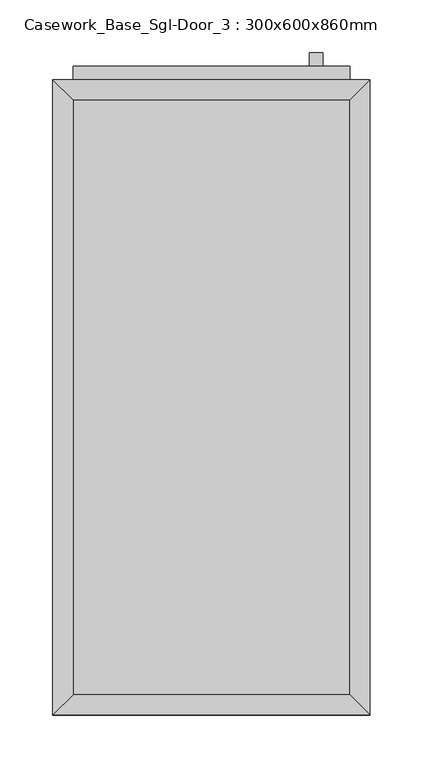
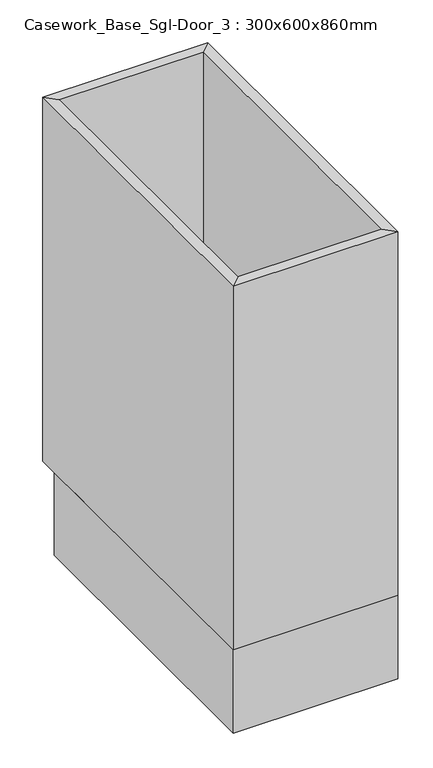
"""IFC4 building model written with IfcOpenShell, lengths in millimetres: furniture geometry, Casework_Base_Sgl-Door_3 : 300x600x860mm."""

import ifcopenshell
import ifcopenshell.guid

model = None  # the IFC model being written
_history = None  # IfcOwnerHistory: only IFC2X3 demands one
_inside = {}  # id of a spatial element -> (the spatial element, [elements in it])
_under = {}  # id of a project, library or spatial element -> (it, [spatial elements below it])
_declared = {}  # id of a project -> (the project, [libraries it declares])
_typed = {}  # id of a type object -> (the type object, [elements of that type])
_made_of = {}  # id of a material, layer set ... -> (it, [elements and type objects made of it])


def new_model(schema):
    """Start an empty IFC model of exactly this schema.

    Asked for "IFC4X3", IfcOpenShell would pick the latest addendum, in which some entities
    have other attributes; the version numbers below select the first issue.
    IFC2X3 requires an IfcOwnerHistory on every rooted entity: one is made here for all.
    """
    global model, _history
    if schema == "IFC4X3":
        model = ifcopenshell.file(schema_version=(4, 3, 0, 0))
    else:
        model = ifcopenshell.file(schema=schema)
    _inside.clear()
    _under.clear()
    _declared.clear()
    _typed.clear()
    _made_of.clear()
    _history = None
    if model.schema == "IFC2X3":
        org = make("IfcOrganization", Name="unknown")
        user = make(
            "IfcPersonAndOrganization",
            ThePerson=make("IfcPerson", FamilyName="unknown"),
            TheOrganization=org,
        )
        app = make(
            "IfcApplication",
            ApplicationDeveloper=org,
            Version="unknown",
            ApplicationFullName="unknown",
            ApplicationIdentifier="unknown",
        )
        _history = make(
            "IfcOwnerHistory",
            OwningUser=user,
            OwningApplication=app,
            ChangeAction="ADDED",
            CreationDate=0,
        )
    return model


def make(cls, **values):
    """One entity of the class cls with the attributes given. An attribute that is None is left unset."""
    return model.create_entity(
        cls, **{name: value for name, value in values.items() if value is not None}
    )


def rooted(cls, **values):
    """An entity with a GlobalId (a new one), such as an element, a storey or a relation."""
    return make(cls, GlobalId=ifcopenshell.guid.new(), OwnerHistory=_history, **values)


def si_unit(unit_type, name, prefix=None):
    """IfcSIUnit, for example si_unit("LENGTHUNIT", "METRE", prefix="MILLI")."""
    return make("IfcSIUnit", UnitType=unit_type, Prefix=prefix, Name=name)


def assignment(units):
    """IfcUnitAssignment: the units of a project."""
    return None if units is None else make("IfcUnitAssignment", Units=units)


def point(xyz):
    """IfcCartesianPoint."""
    return None if xyz is None else make("IfcCartesianPoint", Coordinates=xyz)


def direction(xyz):
    """IfcDirection."""
    return None if xyz is None else make("IfcDirection", DirectionRatios=xyz)


def frame(location, z_axis=None, x_axis=None):
    """IfcAxis2Placement3D, a coordinate frame: its origin and axes. An axis left out is left unset."""
    return make(
        "IfcAxis2Placement3D",
        Location=point(location),
        Axis=direction(z_axis),
        RefDirection=direction(x_axis),
    )


def origin():
    """The frame at (0, 0, 0) with its axes left unset."""
    return frame((0.0, 0.0, 0.0))


def origin_with_axes():
    """The frame at (0, 0, 0) with the z axis (0, 0, 1) and the x axis (1, 0, 0) written out."""
    return frame((0.0, 0.0, 0.0), z_axis=(0.0, 0.0, 1.0), x_axis=(1.0, 0.0, 0.0))


def place(relative_to, where):
    """IfcLocalPlacement: puts the frame where relative to a parent placement (None: the world)."""
    return make(
        "IfcLocalPlacement", PlacementRelTo=relative_to, RelativePlacement=where
    )


def context(
    kind, dimensions, precision=None, world=None, true_north=None, identifier=None
):
    """IfcGeometricRepresentationContext, for example the 3D "Model" context."""
    return make(
        "IfcGeometricRepresentationContext",
        ContextIdentifier=identifier,
        ContextType=kind,
        CoordinateSpaceDimension=dimensions,
        Precision=precision,
        WorldCoordinateSystem=world,
        TrueNorth=true_north,
    )


def project(units=None, contexts=None):
    """IfcProject with its units and contexts."""
    return rooted(
        "IfcProject",
        Name="project",
        RepresentationContexts=contexts,
        UnitsInContext=assignment(units),
    )


def spatial(cls, under=None, at=None, **own):
    """A site, building, storey or space (cls), placed at a placement, below another one or the project."""
    s = rooted(cls, ObjectPlacement=at, **own)
    if under is not None:
        _under.setdefault(under.id(), (under, []))[1].append(s)
    return s


def polyline(points):
    """IfcPolyline through the points."""
    return make("IfcPolyline", Points=[point(p) for p in points])


def outline(outer, holes=None, kind="AREA"):
    """IfcArbitraryClosedProfileDef: a profile drawn as a closed curve; with holes, ...WithVoids."""
    if holes is None:
        return make("IfcArbitraryClosedProfileDef", ProfileType=kind, OuterCurve=outer)
    return make(
        "IfcArbitraryProfileDefWithVoids",
        ProfileType=kind,
        OuterCurve=outer,
        InnerCurves=holes,
    )


def extrude(swept, where, along, depth):
    """IfcExtrudedAreaSolid: the profile swept, set in the frame where, extruded along a direction by depth."""
    return make(
        "IfcExtrudedAreaSolid",
        SweptArea=swept,
        Position=where,
        ExtrudedDirection=direction(along),
        Depth=depth,
    )


def faces_of(points, faces, orient=None, outer=None):
    """IfcFace entities. A face is a list of loops; a loop is a list of indices into points, from 0.

    orient and outer hold one flag for each loop. By default every Orientation is true, the
    first loop of a face is its IfcFaceOuterBound and the others are IfcFaceBound.
    """
    made = []
    for i, loops in enumerate(faces):
        bounds = []
        for j, loop in enumerate(loops):
            is_outer = j == 0 if outer is None else outer[i][j]
            bounds.append(
                make(
                    "IfcFaceOuterBound" if is_outer else "IfcFaceBound",
                    Bound=make("IfcPolyLoop", Polygon=[points[k] for k in loop]),
                    Orientation=True if orient is None else orient[i][j],
                )
            )
        made.append(make("IfcFace", Bounds=bounds))
    return made


def faceted_brep(points, faces, orient=None, outer=None, voids=None):
    """IfcFacetedBrep: a solid bounded by flat faces; with voids (closed shells), ...WithVoids."""
    shared = [point(p) for p in points]
    hull = make("IfcClosedShell", CfsFaces=faces_of(shared, faces, orient, outer))
    if voids is None:
        return make("IfcFacetedBrep", Outer=hull)
    return make(
        "IfcFacetedBrepWithVoids",
        Outer=hull,
        Voids=[
            make(cls, CfsFaces=faces_of(shared, fs, o, b)) for cls, fs, o, b in voids
        ],
    )


def shape(context_of_items, identifier, shape_type, items):
    """IfcShapeRepresentation: the items that make up one representation, for example the "Body"."""
    return make(
        "IfcShapeRepresentation",
        ContextOfItems=context_of_items,
        RepresentationIdentifier=identifier,
        RepresentationType=shape_type,
        Items=items,
    )


def source(mapping_origin, context_of_items, identifier, shape_type, items):
    """IfcRepresentationMap: a shape defined once, which mapped items show again and again."""
    return make(
        "IfcRepresentationMap",
        MappingOrigin=mapping_origin,
        MappedRepresentation=shape(context_of_items, identifier, shape_type, items),
    )


def transform(
    local_origin,
    x_axis=None,
    y_axis=None,
    z_axis=None,
    scale=None,
    scale2=None,
    scale3=None,
    uniform=True,
):
    """IfcCartesianTransformationOperator3D, or its non-uniform kind. x_axis, y_axis, z_axis: its Axis1, 2, 3."""
    if uniform:
        return make(
            "IfcCartesianTransformationOperator3D",
            Axis1=direction(x_axis),
            Axis2=direction(y_axis),
            LocalOrigin=point(local_origin),
            Scale=scale,
            Axis3=direction(z_axis),
        )
    return make(
        "IfcCartesianTransformationOperator3DnonUniform",
        Axis1=direction(x_axis),
        Axis2=direction(y_axis),
        LocalOrigin=point(local_origin),
        Scale=scale,
        Axis3=direction(z_axis),
        Scale2=scale2,
        Scale3=scale3,
    )


def mapped(mapping_source, mapping_target):
    """IfcMappedItem: shows the shape of a source again, moved by a transform."""
    return make(
        "IfcMappedItem", MappingSource=mapping_source, MappingTarget=mapping_target
    )


def made_of(thing, what):
    """Note that an element or type object is made of a material, layer set ...; save() writes the relation."""
    if what is not None:
        _made_of.setdefault(what.id(), (what, []))[1].append(thing)
    return thing


def element(
    cls,
    number,
    at=None,
    inside=None,
    cuts=None,
    type_object=None,
    material=None,
    context=None,
    identifier="Body",
    shape_type=None,
    held_by="IfcProductDefinitionShape",
    body=None,
    shapes=None,
    **own,
):
    """One element of the class cls, such as IfcWall. Its Tag is "e" and its number.

    at: its placement. inside: the storey or other place that contains it. cuts: it is an
    opening in that element (IfcRelVoidsElement). A single representation is given by context,
    identifier, shape_type and body (its items); several are given by shapes. held_by: the class
    of the entity that holds the representations. save() writes the other relations.
    """
    e = rooted(cls, Tag="e%d" % number, ObjectPlacement=at, **own)
    if body is not None:
        shapes = [shape(context, identifier, shape_type, body)]
    if shapes is not None:
        e.Representation = make(held_by, Representations=shapes)
    if inside is not None:
        _inside.setdefault(inside.id(), (inside, []))[1].append(e)
    if cuts is not None:
        rooted(
            "IfcRelVoidsElement", RelatingBuildingElement=cuts, RelatedOpeningElement=e
        )
    if type_object is not None:
        _typed.setdefault(type_object.id(), (type_object, []))[1].append(e)
    return made_of(e, material)


def aggregate(whole, parts):
    """IfcRelAggregates: a whole, such as a stair, and the parts it consists of."""
    return rooted("IfcRelAggregates", RelatingObject=whole, RelatedObjects=parts)


def save(model, path):
    """Write the relations noted so far, then the file.

    IfcRelAggregates (storeys below a building ...), IfcRelContainedInSpatialStructure (elements
    in a storey), IfcRelDefinesByType, IfcRelAssociatesMaterial and IfcRelDeclares: one each for
    every whole, place, type object, material and project.
    """
    for whole, parts in _under.values():
        aggregate(whole, parts)
    for where, things in _inside.values():
        rooted(
            "IfcRelContainedInSpatialStructure",
            RelatedElements=things,
            RelatingStructure=where,
        )
    for kind, things in _typed.values():
        rooted("IfcRelDefinesByType", RelatedObjects=things, RelatingType=kind)
    for what, things in _made_of.values():
        rooted("IfcRelAssociatesMaterial", RelatedObjects=things, RelatingMaterial=what)
    for by, libraries in _declared.values():
        rooted("IfcRelDeclares", RelatingContext=by, RelatedDefinitions=libraries)
    model.write(path)


def casework_base_sgl_door_3_300x600x860mm_7fc0b309(model_context):
    return source(origin(), model_context, "Body", "SolidModel", [
        extrude(outline(polyline([(149.6877049, 19.05), (-112.2122951, 19.05), (-112.2122951, 580.95), (149.6877049, 580.95), (149.6877049, 19.05)])), frame((0.0, 0.0, 160.0), z_axis=(0.0, 0.0, 1.0), x_axis=(1.0, 0.0, 0.0)), (0.0, 0.0, 1.0), 19.05),
        faceted_brep([(149.6877049, 580.95, 860.0), (-112.2122951, 580.95, 860.0), (-112.2122951, 580.95, 160.0), (149.6877049, 580.95, 160.0), (168.7377049, 600.0, 860.0), (-131.2622951, 600.0, 860.0), (168.7377049, 600.0, 160.0), (-131.2622951, 600.0, 160.0), (-112.2122951, 19.05, 860.0), (-112.2122951, 19.05, 160.0), (-131.2622951, 0.0, 860.0), (-131.2622951, 0.0, 160.0), (149.6877049, 19.05, 860.0), (149.6877049, 19.05, 160.0), (168.7377049, 0.0, 860.0), (168.7377049, 0.0, 160.0)], [[[0, 1, 2, 3]], [[4, 5, 1, 0]], [[6, 7, 5, 4]], [[3, 2, 7, 6]], [[1, 8, 9, 2]], [[5, 10, 8, 1]], [[7, 11, 10, 5]], [[2, 9, 11, 7]], [[8, 12, 13, 9]], [[10, 14, 12, 8]], [[11, 15, 14, 10]], [[9, 13, 15, 11]], [[12, 0, 3, 13]], [[14, 4, 0, 12]], [[15, 6, 4, 14]], [[13, 3, 6, 15]]]),
        extrude(outline(polyline([(168.7377049, 0.0), (-131.2622951, 0.0), (-131.2622951, 565.0), (168.7377049, 565.0), (168.7377049, 0.0)])), origin_with_axes(), (0.0, 0.0, 1.0), 160.0),
        extrude(outline(polyline([(124.2877049, 625.4), (124.2877049, 612.7), (111.5877049, 612.7), (111.5877049, 625.4), (124.2877049, 625.4)])), frame((0.0, 0.0, 701.25), z_axis=(0.0, 0.0, 1.0), x_axis=(1.0, 0.0, 0.0)), (0.0, 0.0, 1.0), 101.6),
        extrude(outline(polyline([(149.6877049, 612.7), (149.6877049, 600.0), (-112.2122951, 600.0), (-112.2122951, 612.7), (149.6877049, 612.7)])), frame((0.0, 0.0, 179.05), z_axis=(0.0, 0.0, 1.0), x_axis=(1.0, 0.0, 0.0)), (0.0, 0.0, 1.0), 661.9),
    ])


if __name__ == "__main__":
    model = new_model("IFC4")
    model_context = context("Model", 3, world=origin())
    ifc_project = project(units=[si_unit("LENGTHUNIT", "METRE", prefix="MILLI")], contexts=[model_context])
    site = spatial("IfcSite", under=ifc_project)
    building = spatial("IfcBuilding", under=site)
    placement = place(None, origin())
    casework_base_sgl_door_3_300x600x860mm_shape = casework_base_sgl_door_3_300x600x860mm_7fc0b309(model_context)
    element("IfcFurniture", 1, ObjectType="Casework_Base_Sgl-Door_3 : 300x600x860mm", at=placement, inside=building, context=model_context, shape_type="MappedRepresentation", body=[
        mapped(casework_base_sgl_door_3_300x600x860mm_shape, transform((0.0, 0.0, 0.0), x_axis=(1.0, 0.0, 0.0), y_axis=(0.0, 1.0, 0.0), z_axis=(0.0, 0.0, 1.0))),
    ])
    save(model, "model.ifc")

# Revit data of these elements
# Type "Casework_Base_Sgl-Door_3 : 300x600x860mm"
#   Keynote = "N10"
#   Depth = 600 mm
#   Height = 860 mm
#   Plinth Depth = 35 mm
#   Plinth Height = 160 mm
#   Width = 300 mm
#   Material Cabinet = Cabinets
#   Material Door/Drawer = Cabinets
#   Material Handle = Cabinets - Handles
#   Default Elevation = 0
# Element 1 (IfcFurniture, "Casework_Base_Sgl-Door_3 : 300x600x860mm")
#   Materials on its faces: "Cabinets", "Cabinets - Handles"
# Materials
#   "Cabinets": class "Miscellaneous", colour RGB 249 249 249, transparency 0
#   "Cabinets - Handles": class "Metal", colour RGB 57 57 57, transparency 0
